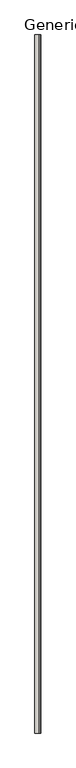
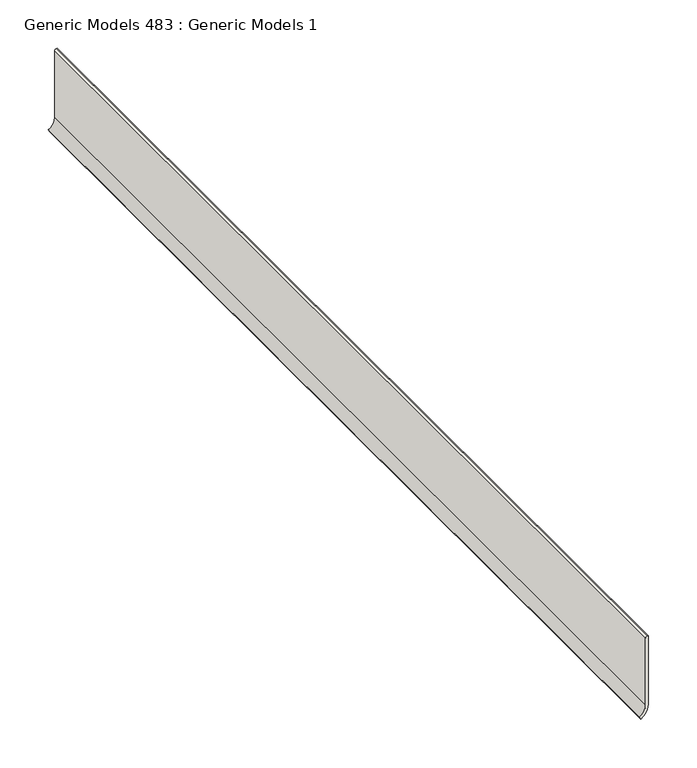
"""IFC4 building model written with IfcOpenShell, lengths in millimetres: wall geometry, Generic Models 483 : Generic Models 1."""

from ifc_helpers import new_model, si_unit, point, frame, frame_2d, origin, place, context, project, spatial, polyline, circle_curve, trimmed, segment, composite_curve, outline, extrude, source, transform, mapped, element, save


def generic_models_483_generic_models_1_48395e05(model_context):
    return source(origin(), model_context, "Body", "SweptSolid", [
        extrude(outline(composite_curve([segment(polyline([(101.6, 141075.2886541), (101.6, 141074.2004559)]), True, "CONTINUOUS"), segment(trimmed(circle_curve(frame_2d((99.5131982, 141074.2004559)), 2.0868018), [point((101.6, 141074.2004559))], [point((99.5131982, 141072.1136541))], False, "CARTESIAN"), True, "CONTINUOUS"), segment(polyline([(99.5131982, 141072.1136541), (15.4496307, 141072.1136541)]), True, "CONTINUOUS"), segment(trimmed(circle_curve(frame_2d((15.4496307, 141057.4489572)), 14.6646968), [point((15.4496307, 141072.1136541))], [point((2.7496307, 141064.7813057))], True, "CARTESIAN"), True, "CONTINUOUS"), segment(polyline([(2.7496307, 141064.7813057), (0.0, 141066.3688057)]), True, "CONTINUOUS"), segment(trimmed(circle_curve(frame_2d((15.4496307, 141057.4489572)), 17.8396968), [point((0.0, 141066.3688057))], [point((15.4496307, 141075.2886541))], False, "CARTESIAN"), True, "CONTINUOUS"), segment(polyline([(15.4496307, 141075.2886541), (101.6, 141075.2886541)]), True, "CONTINUOUS")], self_intersect=False)), frame((0.0, 0.0, 0.0), z_axis=(0.0, 1.0, 0.0), x_axis=(0.0, 0.0, 1.0)), (0.0, 0.0, 1.0), 1219.2),
    ])


if __name__ == "__main__":
    model = new_model("IFC4")
    model_context = context("Model", 3, world=origin())
    ifc_project = project(units=[si_unit("LENGTHUNIT", "METRE", prefix="MILLI")], contexts=[model_context])
    site = spatial("IfcSite", under=ifc_project)
    building = spatial("IfcBuilding", under=site)
    placement = place(None, origin())
    generic_models_483_generic_models_1_shape = generic_models_483_generic_models_1_48395e05(model_context)
    element("IfcWall", 1, ObjectType="Generic Models 483 : Generic Models 1", at=placement, inside=building, context=model_context, shape_type="MappedRepresentation", body=[
        mapped(generic_models_483_generic_models_1_shape, transform((0.0, 0.0, 0.0), x_axis=(1.0, 0.0, 0.0), y_axis=(0.0, 1.0, 0.0), z_axis=(0.0, 0.0, 1.0))),
    ])
    save(model, "model.ifc")

# Revit data of these elements
# Element 1 (IfcWall, "Generic Models 483 : Generic Models 1")
#   Materials on its faces: "WALL BASE AS SCHEDULED"
# Materials
#   "WALL BASE AS SCHEDULED": class "Generic", colour RGB 120 120 120, transparency 0, Cost = 0
